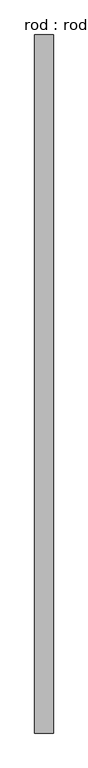
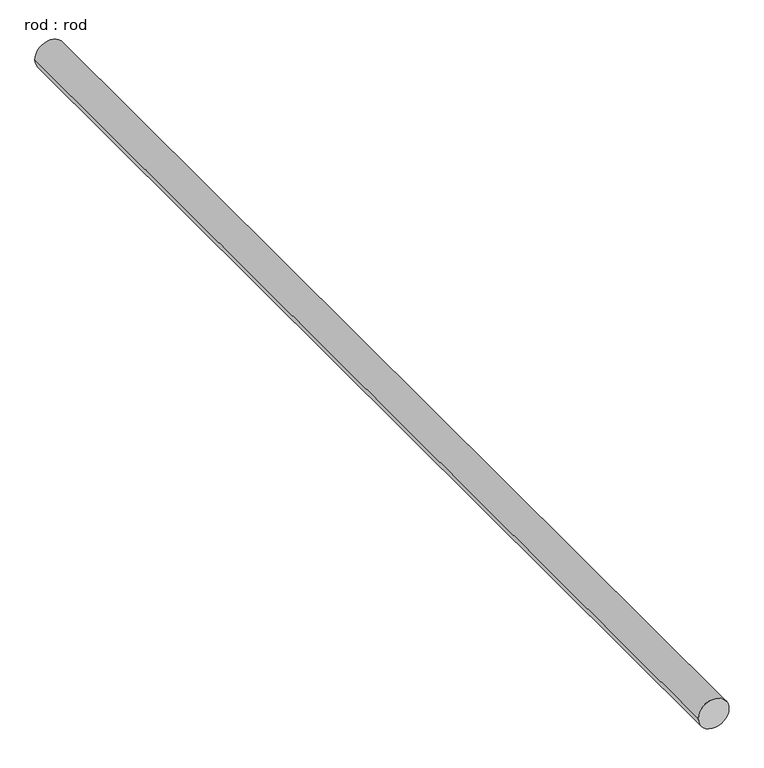
"""IFC4 building model written with IfcOpenShell, lengths in millimetres: proxy geometry, rod : rod."""

from ifc_helpers import new_model, si_unit, point, frame, frame_2d, origin, place, context, project, spatial, circle_curve, trimmed, segment, composite_curve, outline, extrude, source, transform, mapped, element, save


def rod_rod_8b19b318(model_context):
    return source(origin(), model_context, "Body", "SweptSolid", [
        extrude(outline(composite_curve([segment(trimmed(circle_curve(frame_2d((0.0108462, 0.0)), 200.0), [point((0.0108462, 200.0))], [point((0.0108462, -200.0))], False, "CARTESIAN"), True, "CONTINUOUS"), segment(trimmed(circle_curve(frame_2d((0.0108462, 0.0)), 200.0), [point((0.0108462, -200.0))], [point((0.0108462, 200.0))], False, "CARTESIAN"), True, "CONTINUOUS")], self_intersect=False)), frame((0.0, -3402.0733333, 0.0), z_axis=(0.0, 1.0, 0.0), x_axis=(0.0, 0.0, 1.0)), (0.0, 0.0, 1.0), 14989.6038974),
    ])


if __name__ == "__main__":
    model = new_model("IFC4")
    model_context = context("Model", 3, world=origin())
    ifc_project = project(units=[si_unit("LENGTHUNIT", "METRE", prefix="MILLI")], contexts=[model_context])
    site = spatial("IfcSite", under=ifc_project)
    building = spatial("IfcBuilding", under=site)
    placement = place(None, origin())
    rod_rod_shape = rod_rod_8b19b318(model_context)
    element("IfcBuildingElementProxy", 1, Name="rod : rod", ObjectType="rod : rod", at=placement, inside=building, context=model_context, shape_type="MappedRepresentation", body=[
        mapped(rod_rod_shape, transform((0.0, 0.0, 0.0), x_axis=(1.0, 0.0, 0.0), y_axis=(0.0, 1.0, 0.0), z_axis=(0.0, 0.0, 1.0))),
    ])
    save(model, "model.ifc")

# Revit data of these elements
# Type "rod : rod"
#   Default Elevation = 0
